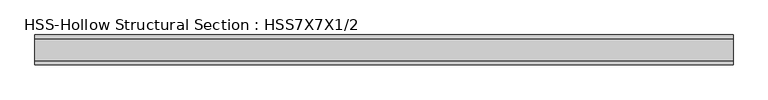
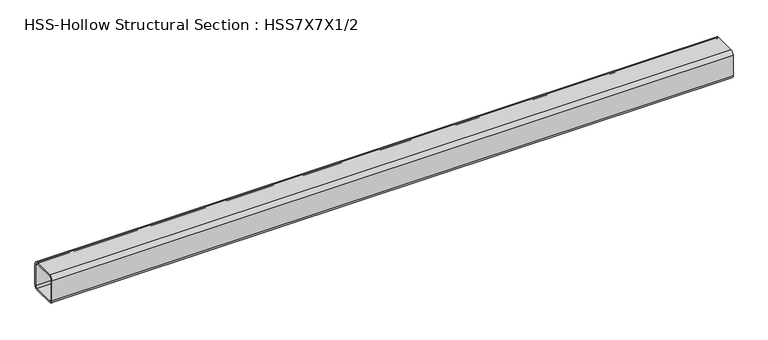
"""IFC4 building model written with IfcOpenShell, lengths in millimetres: member geometry, HSS-Hollow Structural Section : HSS7X7X1/2."""

from ifc_helpers import new_model, si_unit, point, frame, frame_2d, origin, place, context, project, spatial, polyline, circle_curve, trimmed, segment, composite_curve, outline, extrude, source, transform, mapped, element, save


def hss_hollow_structural_section_hss7x7x1_2_aaab51d8(model_context):
    return source(origin(), model_context, "Body", "SweptSolid", [
        extrude(outline(composite_curve([segment(polyline([(88.9, 65.278), (88.9, -65.278)]), True, "CONTINUOUS"), segment(trimmed(circle_curve(frame_2d((65.278, -65.278)), 23.622), [point((88.9, -65.278))], [point((65.278, -88.9))], False, "CARTESIAN"), True, "CONTINUOUS"), segment(polyline([(65.278, -88.9), (-65.278, -88.9)]), True, "CONTINUOUS"), segment(trimmed(circle_curve(frame_2d((-65.278, -65.278)), 23.622), [point((-65.278, -88.9))], [point((-88.9, -65.278))], False, "CARTESIAN"), True, "CONTINUOUS"), segment(polyline([(-88.9, -65.278), (-88.9, 65.278)]), True, "CONTINUOUS"), segment(trimmed(circle_curve(frame_2d((-65.278, 65.278)), 23.622), [point((-88.9, 65.278))], [point((-65.278, 88.9))], False, "CARTESIAN"), True, "CONTINUOUS"), segment(polyline([(-65.278, 88.9), (65.278, 88.9)]), True, "CONTINUOUS"), segment(trimmed(circle_curve(frame_2d((65.278, 65.278)), 23.622), [point((65.278, 88.9))], [point((88.9, 65.278))], False, "CARTESIAN"), True, "CONTINUOUS")], self_intersect=False), holes=[composite_curve([segment(trimmed(circle_curve(frame_2d((-65.278, 65.278)), 11.811), [point((-65.278, 77.089))], [point((-77.089, 65.278))], True, "CARTESIAN"), True, "CONTINUOUS"), segment(polyline([(-77.089, 65.278), (-77.089, -65.278)]), True, "CONTINUOUS"), segment(trimmed(circle_curve(frame_2d((-65.278, -65.278)), 11.811), [point((-77.089, -65.278))], [point((-65.278, -77.089))], True, "CARTESIAN"), True, "CONTINUOUS"), segment(polyline([(-65.278, -77.089), (65.278, -77.089)]), True, "CONTINUOUS"), segment(trimmed(circle_curve(frame_2d((65.278, -65.278)), 11.811), [point((65.278, -77.089))], [point((77.089, -65.278))], True, "CARTESIAN"), True, "CONTINUOUS"), segment(polyline([(77.089, -65.278), (77.089, 65.278)]), True, "CONTINUOUS"), segment(trimmed(circle_curve(frame_2d((65.278, 65.278)), 11.811), [point((77.089, 65.278))], [point((65.278, 77.089))], True, "CARTESIAN"), True, "CONTINUOUS"), segment(polyline([(65.278, 77.089), (-65.278, 77.089)]), True, "CONTINUOUS")], self_intersect=False)]), frame((-2171.9784546, 0.0, 0.0), z_axis=(1.0, 0.0, 0.0), x_axis=(0.0, 1.0, 0.0)), (0.0, 0.0, 1.0), 4126.0309082),
    ])


if __name__ == "__main__":
    model = new_model("IFC4")
    model_context = context("Model", 3, world=origin())
    ifc_project = project(units=[si_unit("LENGTHUNIT", "METRE", prefix="MILLI")], contexts=[model_context])
    site = spatial("IfcSite", under=ifc_project)
    building = spatial("IfcBuilding", under=site)
    placement = place(None, origin())
    hss_hollow_structural_section_hss7x7x1_2_shape = hss_hollow_structural_section_hss7x7x1_2_aaab51d8(model_context)
    element("IfcMember", 1, ObjectType="HSS-Hollow Structural Section : HSS7X7X1/2", at=placement, inside=building, context=model_context, shape_type="MappedRepresentation", body=[
        mapped(hss_hollow_structural_section_hss7x7x1_2_shape, transform((0.0, 0.0, 0.0), x_axis=(1.0, 0.0, 0.0), y_axis=(0.0, 1.0, 0.0), z_axis=(0.0, 0.0, 1.0))),
    ])
    save(model, "model.ifc")

# Revit data of these elements
# Type "HSS-Hollow Structural Section : HSS7X7X1/2"
#   Assembly Code = "B10"
#   Shape = "Square"
#   W = 41.9
#   Ht = 0' - 7"
#   Length [instance default] = 5' - 0"
#   b = 0' - 7"
#   kr = 0' - 0.93"
#   t = 0' - 0.465"
#   A = 0.0805556 SF
#   Structural Material [instance default] = Steel ASTM A500, Grade B, Rectangular and Square
# Element 1 (IfcMember, "HSS-Hollow Structural Section : HSS7X7X1/2")
#   Materials on its faces: "Steel ASTM A500, Grade B, Rectangular and Square"
# Materials
#   "Steel ASTM A500, Grade B, Rectangular and Square": class "Metal", colour RGB 199 199 199, transparency 0, Description = "Carbon steel", Cost = 0
